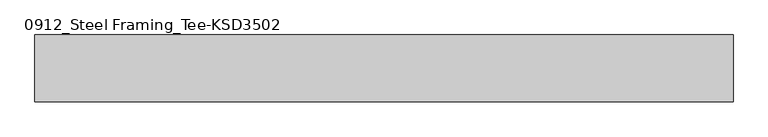
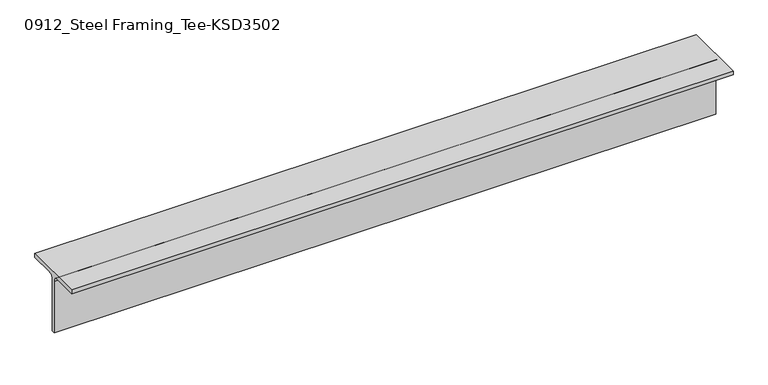
"""IFC4 building model written with IfcOpenShell, lengths in millimetres: member geometry, 0912_Steel Framing_Tee-KSD3502 : H_SB_ASB_CT-150x150x6.5x9."""

from ifc_helpers import new_model, si_unit, point, frame, frame_2d, origin, place, context, project, spatial, polyline, circle_curve, trimmed, segment, composite_curve, outline, extrude, source, transform, mapped, element, save


def member_0912_steel_framing_tee_ksd3502_252e05dd(model_context):
    return source(origin(), model_context, "Body", "SweptSolid", [
        extrude(outline(composite_curve([segment(polyline([(-75.0, 75.0), (75.0, 75.0), (75.0, 66.0), (16.25, 66.0)]), True, "CONTINUOUS"), segment(trimmed(circle_curve(frame_2d((16.25, 53.0)), 13.0), [point((16.25, 66.0))], [point((3.25, 53.0))], True, "CARTESIAN"), True, "CONTINUOUS"), segment(polyline([(3.25, 53.0), (3.25, -75.0), (-3.25, -75.0), (-3.25, 53.0)]), True, "CONTINUOUS"), segment(trimmed(circle_curve(frame_2d((-16.25, 53.0)), 13.0), [point((-3.25, 53.0))], [point((-16.25, 66.0))], True, "CARTESIAN"), True, "CONTINUOUS"), segment(polyline([(-16.25, 66.0), (-75.0, 66.0), (-75.0, 75.0)]), True, "CONTINUOUS")], self_intersect=False)), frame((-860.2, 0.0, 0.0), z_axis=(1.0, 0.0, 0.0), x_axis=(0.0, 1.0, 0.0)), (0.0, 0.0, 1.0), 1561.9),
    ])


if __name__ == "__main__":
    model = new_model("IFC4")
    model_context = context("Model", 3, world=origin())
    ifc_project = project(units=[si_unit("LENGTHUNIT", "METRE", prefix="MILLI")], contexts=[model_context])
    site = spatial("IfcSite", under=ifc_project)
    building = spatial("IfcBuilding", under=site)
    placement = place(None, origin())
    member_0912_steel_framing_tee_ksd3502_shape = member_0912_steel_framing_tee_ksd3502_252e05dd(model_context)
    element("IfcMember", 1, ObjectType="0912_Steel Framing_Tee-KSD3502 : H_SB_ASB_CT-150x150x6.5x9", at=placement, inside=building, context=model_context, shape_type="MappedRepresentation", body=[
        mapped(member_0912_steel_framing_tee_ksd3502_shape, transform((0.0, 0.0, 0.0), x_axis=(1.0, 0.0, 0.0), y_axis=(0.0, 1.0, 0.0), z_axis=(0.0, 0.0, 1.0))),
    ])
    save(model, "model.ifc")

# Revit data of these elements
# Type "0912_Steel Framing_Tee-KSD3502 : H_SB_ASB_CT-150x150x6.5x9"
#   H_WM Code_1 = "S01AA003-00001 | Main Steel Structure Fabrication Work | Shelter/Building | Light Steel - Standard (30KG/M>Weight) | Material: (   )"
#   H_WM Code_2 = "S03AA029-00001 | Main Steel Structure Erection Work | Shelter/Building | Light Steel (30KG/M>Weight) | Material: (   )"
#   H_WM Code_3 = "S01AA010-00001 | Main Steel Structure Fabrication Work | Shelter/Building | Steel Painting/Coating | for Non-Fireproofed Steel Surface, Surface Preparation, Primer, Second & Final Coat | Material: (   )"
#   H_Q'ty Cal Type Tag = "SB-Q2"
#   Width = 15.0 cm
#   Web Thickness = 0.65 cm
#   Web Fillet = 1.3 cm
#   Section Area = 23.39 cm²
#   Perimeter = 0.60 m²/m
#   Nominal Weight = 18.40 kgf/m
#   Height = 15.0 cm
#   Flange Thickness = 0.9 cm
#   Centroid Vertical = 7.5 cm
#   Centroid Horizontal = 7.5 cm
#   Length [instance default] = 1.5000 m
#   Structural Material [instance default] = Steel, 45-345
#   Warping Constant = (empty or 0)
#   Torsional Moment of Inertia = 0
#   Section Name Key = ""
#   Plastic Modulus weak axis = 0
#   Plastic Modulus strong axis = 0
#   Moment of Inertia weak axis = 0
#   Moment of Inertia strong axis = 0
#   Elastic Modulus weak axis = 0
#   Elastic Modulus strong axis = 0
#   Bolt Spacing = 0
#   Assembly Code = ""
# Element 1 (IfcMember, "0912_Steel Framing_Tee-KSD3502 : H_SB_ASB_CT-150x150x6.5x9")
#   Structural Material = none
# Materials
#   "Steel, 45-345": class "Metal", colour RGB 189 187 185, transparency 0, Description = "Steel 345 MPa", Cost = 0
